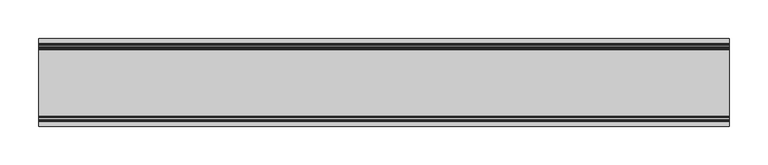
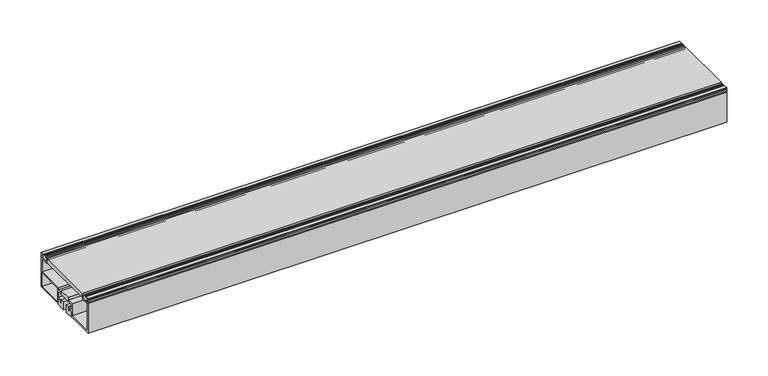
"""IFC4 building model written with IfcOpenShell, lengths in millimetres: proxy geometry, Generic Models 3:Generic Models 1:2:Generic Models 1:2 : Generic Models 3:Generic Models 1:300625:328150:Generic Models 1:2:Generic Models 1:2 : Generic Models 3:Generic Models 1:300625:328150 : Generic Models 3:Generic Models 1:2:Generic Models 1:2 : Generic Models 3:Generic Models 1:300625:328150:4 : Generic Models 3:Generic Models 1:2:Generic Models 1:2 : Generic Models 3:Generic Models 1:300625:328150:Generic Models 1:2:Generic Models 1:2 : Generic Models 3:Generic Models 1:300625:328150 : Generic Models 3:Generic Models 1:2:Generic Models 1:2 : Generic Models 3:Generic Models 1:300625:328150:300962."""

from ifc_helpers import new_model, si_unit, frame, origin, place, context, project, spatial, polyline, outline, extrude, source, transform, mapped, element, save


def generic_models_bcc34015(model_context):
    return source(origin(), model_context, "Body", "SweptSolid", [
        extrude(outline(polyline([(-568050.8100714, 2442.2790126), (-568047.9643932, 2442.2790126), (-568047.9643932, 2445.2228723), (-568043.6663214, 2445.2228723), (-568043.6663214, 2437.3831629), (-568055.5641272, 2435.9222961), (-568055.5641272, 2447.9925532), (-568050.8100714, 2447.9925532), (-568050.8100714, 2442.2790126)])), frame((592836.3867242, 0.0, 0.0), z_axis=(1.0, 0.0, 0.0), x_axis=(0.0, 1.0, 0.0)), (0.0, 0.0, 1.0), 895.35),
        extrude(outline(polyline([(593731.7367242, -568016.9406051), (593731.7367242, -568102.342163), (592836.3867242, -568102.342163), (592836.3867242, -568016.9406051), (593731.7367242, -568016.9406051)])), frame((0.0, 0.0, 2482.8143609), z_axis=(0.0, 0.0, 1.0), x_axis=(1.0, 0.0, 0.0)), (0.0, 0.0, 1.0), 6.35),
        extrude(outline(polyline([(-568002.371855, 2483.7801242), (-568001.9944464, 2482.8143609), (-568007.8625385, 2482.8143609), (-568006.2693218, 2483.6971498), (-568005.2951168, 2484.9385339), (-568005.0923289, 2486.3443102), (-568005.6926824, 2487.6945579), (-568007.0022575, 2488.7780434), (-568007.8625385, 2489.1643609), (-568001.9944464, 2489.1643609), (-568002.371855, 2488.1985977), (-568002.6855411, 2485.9893609), (-568002.371855, 2483.7801242)])), frame((592836.3867242, 0.0, 0.0), z_axis=(1.0, 0.0, 0.0), x_axis=(0.0, 1.0, 0.0)), (0.0, 0.0, 1.0), 895.35),
        extrude(outline(polyline([(-568005.9353019, 2487.3669418), (-568005.4636661, 2485.9893609), (-568005.9353019, 2484.6117801), (-568007.2567959, 2483.507046), (-568009.1664101, 2482.8939648), (-568010.2261661, 2482.8143609), (-568011.285922, 2482.8939648), (-568013.1955363, 2483.507046), (-568014.5170303, 2484.6117801), (-568014.9886661, 2485.9893609), (-568014.5170303, 2487.3669418), (-568013.1955363, 2488.4716759), (-568011.285922, 2489.0847571), (-568010.2261661, 2489.1643609), (-568009.1664101, 2489.0847571), (-568007.2567959, 2488.4716759), (-568005.9353019, 2487.3669418)])), frame((592836.3867242, 0.0, 0.0), z_axis=(1.0, 0.0, 0.0), x_axis=(0.0, 1.0, 0.0)), (0.0, 0.0, 1.0), 895.35),
        extrude(outline(polyline([(-568107.0029708, 2489.0847571), (-568105.0933565, 2488.4716759), (-568103.7718625, 2487.3669418), (-568103.3002267, 2485.9893609), (-568103.7718625, 2484.6117801), (-568105.0933565, 2483.507046), (-568107.0029708, 2482.8939648), (-568108.0627267, 2482.8143609), (-568109.1224826, 2482.8939648), (-568111.0320969, 2483.507046), (-568112.3535909, 2484.6117801), (-568112.8252267, 2485.9893609), (-568112.3535909, 2487.3669418), (-568111.0320969, 2488.4716759), (-568109.1224826, 2489.0847571), (-568108.0627267, 2489.1643609), (-568107.0029708, 2489.0847571)])), frame((592836.3867242, 0.0, 0.0), z_axis=(1.0, 0.0, 0.0), x_axis=(0.0, 1.0, 0.0)), (0.0, 0.0, 1.0), 895.35),
        extrude(outline(polyline([(-568110.4263543, 2489.1643609), (-568111.2866352, 2488.7780434), (-568112.5962104, 2487.6945579), (-568113.1965639, 2486.3443102), (-568112.993776, 2484.9385339), (-568112.019571, 2483.6971498), (-568110.4263543, 2482.8143609), (-568116.2944464, 2482.8143609), (-568115.9170378, 2483.7801242), (-568115.6033517, 2485.9893609), (-568115.9170378, 2488.1985977), (-568116.2944464, 2489.1643609), (-568110.4263543, 2489.1643609)])), frame((592836.3867242, 0.0, 0.0), z_axis=(1.0, 0.0, 0.0), x_axis=(0.0, 1.0, 0.0)), (0.0, 0.0, 1.0), 895.35),
        extrude(outline(polyline([(593731.7367242, -568050.8100714), (593731.7367242, -568067.4788214), (592836.3867242, -568067.4788214), (592836.3867242, -568050.8100714), (593731.7367242, -568050.8100714)])), frame((0.0, 0.0, 2456.2167541), z_axis=(0.0, 0.0, 1.0), x_axis=(1.0, 0.0, 0.0)), (0.0, 0.0, 1.0), 5.5626),
        extrude(outline(polyline([(-568067.4788214, 2442.2790126), (-568067.4788214, 2447.9925532), (-568062.7247655, 2447.9925532), (-568062.7247655, 2435.9222961), (-568074.6225714, 2437.3831629), (-568074.6225714, 2445.2228723), (-568070.3244996, 2445.2228723), (-568070.3244996, 2442.2790126), (-568067.4788214, 2442.2790126)])), frame((592836.3867242, 0.0, 0.0), z_axis=(1.0, 0.0, 0.0), x_axis=(0.0, 1.0, 0.0)), (0.0, 0.0, 1.0), 895.35),
        extrude(outline(polyline([(-568116.2944464, 2482.8162234), (-568103.2073153, 2482.8162234), (-568103.2073153, 2480.9162899), (-568113.7865342, 2480.9162899), (-568113.7865342, 2440.2999335), (-568076.8779936, 2440.2999335), (-568076.8779936, 2458.1166876), (-568043.3108327, 2458.1166876), (-568043.3108327, 2461.7031541), (-568004.5023586, 2461.7031541), (-568004.5023586, 2480.9162899), (-568015.0815775, 2480.9162899), (-568015.0815775, 2482.8162234), (-568001.9944464, 2482.8162234), (-568001.9944464, 2438.4), (-568043.3108327, 2438.4), (-568043.3108327, 2445.6197473), (-568048.4026545, 2445.6197473), (-568048.4026545, 2442.6758876), (-568050.4545827, 2442.6758876), (-568050.4545827, 2447.5956782), (-568043.3108327, 2447.5956782), (-568043.3108327, 2456.2167541), (-568074.9780601, 2456.2167541), (-568074.9780601, 2447.5956782), (-568067.8343101, 2447.5956782), (-568067.8343101, 2442.6758876), (-568069.8862383, 2442.6758876), (-568069.8862383, 2445.6197473), (-568074.9780601, 2445.6197473), (-568074.9780601, 2438.4), (-568116.2944464, 2438.4), (-568116.2944464, 2482.8162234)]), holes=[polyline([(-568041.4108992, 2459.8032206), (-568041.4108992, 2440.2999335), (-568004.5023586, 2440.2999335), (-568004.5023586, 2459.8032206), (-568041.4108992, 2459.8032206)])]), frame((592836.3867242, 0.0, 0.0), z_axis=(1.0, 0.0, 0.0), x_axis=(0.0, 1.0, 0.0)), (0.0, 0.0, 1.0), 895.35),
    ])


if __name__ == "__main__":
    model = new_model("IFC4")
    model_context = context("Model", 3, world=origin())
    ifc_project = project(units=[si_unit("LENGTHUNIT", "METRE", prefix="MILLI")], contexts=[model_context])
    site = spatial("IfcSite", under=ifc_project)
    building = spatial("IfcBuilding", under=site)
    placement = place(None, origin())
    generic_models_shape = generic_models_bcc34015(model_context)
    element("IfcBuildingElementProxy", 1, Name="Generic Models 3:Generic Models 1:2:Generic Models 1:2 : Generic Models 3:Generic Models 1:300625:328150:Generic Models 1:2:Generic Models 1:2 : Generic Models 3:Generic Models 1:300625:328150 : Generic Models 3:Generic Models 1:2:Generic Models 1:2 : Generic Models 3:Generic Models 1:300625:328150:4 : Generic Models 3:Generic Models 1:2:Generic Models 1:2 : Generic Models 3:Generic Models 1:300625:328150:Generic Models 1:2:Generic Models 1:2 : Generic Models 3:Generic Models 1:300625:328150 : Generic Models 3:Generic Models 1:2:Generic Models 1:2 : Generic Models 3:Generic Models 1:300625:328150:300962", ObjectType="Generic Models 3:Generic Models 1:2:Generic Models 1:2 : Generic Models 3:Generic Models 1:300625:328150:Generic Models 1:2:Generic Models 1:2 : Generic Models 3:Generic Models 1:300625:328150 : Generic Models 3:Generic Models 1:2:Generic Models 1:2 : Generic Models 3:Generic Models 1:300625:328150:4 : Generic Models 3:Generic Models 1:2:Generic Models 1:2 : Generic Models 3:Generic Models 1:300625:328150:Generic Models 1:2:Generic Models 1:2 : Generic Models 3:Generic Models 1:300625:328150 : Generic Models 3:Generic Models 1:2:Generic Models 1:2 : Generic Models 3:Generic Models 1:300625:328150:300962", at=placement, inside=building, context=model_context, shape_type="MappedRepresentation", body=[
        mapped(generic_models_shape, transform((0.0, 0.0, 0.0), x_axis=(1.0, 0.0, 0.0), y_axis=(0.0, 1.0, 0.0), z_axis=(0.0, 0.0, 1.0))),
    ])
    save(model, "model.ifc")

# Revit data of these elements
# Type "Generic Models 3:Generic Models 1:2:Generic Models 1:2 : Generic Models 3:Generic Models 1:300625:328150:Generic Models 1:2:Generic Models 1:2 : Generic Models 3:Generic Models 1:300625:328150 : Generic Models 3:Generic Models 1:2:Generic Models 1:2 : Generic Models 3:Generic Models 1:300625:328150:4 : Generic Models 3:Generic Models 1:2:Generic Models 1:2 : Generic Models 3:Generic Models 1:300625:328150:Generic Models 1:2:Generic Models 1:2 : Generic Models 3:Generic Models 1:300625:328150 : Generic Models 3:Generic Models 1:2:Generic Models 1:2 : Generic Models 3:Generic Models 1:300625:328150:300962"
#   NameOverride = "Generic Models 3:Generic Models 1:2:Generic Models 1:2 : Generic Models 3:Generic Models 1:300625:328150:Generic Models 1:2:Generic Models 1:2 : Generic Models 3:Generic Models 1:300625:328150 : Generic Models 3:Generic Models 1:2:Generic Models 1:2 : Generic Models 3:Generic Models 1:300625:328150:300962"
#   ObjectTypeOverride = "Generic Models 1:2:Generic Models 1:2 : Generic Models 3:Generic Models 1:300625:328150 : Generic Models 3:Generic Models 1:2:Generic Models 1:2 : Generic Models 3:Generic Models 1:300625:328150"
#   Reference = "Generic Models 1"
#   Tag = "300962"
# Element 1 (IfcBuildingElementProxy, "Generic Models 3:Generic Models 1:2:Generic Models 1:2 : Generic Models 3:Generic Models 1:300625:328150:Generic Models 1:2:Generic Models 1:2 : Generic Models 3:Generic Models 1:300625:328150 : Generic Models 3:Generic Models 1:2:Generic Models 1:2 : Generic Models 3:Generic Models 1:300625:328150:4 : Generic Models 3:Generic Models 1:2:Generic Models 1:2 : Generic Models 3:Generic Models 1:300625:328150:Generic Models 1:2:Generic Models 1:2 : Generic Models 3:Generic Models 1:300625:328150 : Generic Models 3:Generic Models 1:2:Generic Models 1:2 : Generic Models 3:Generic Models 1:300625:328150:300962")
#   Materials on its faces: "SEALANT & BACKER ROD, IF NECESSARY", "INTERIOR GRADE ALUMINUM STOREFRONT W/ SINGLE GLAZING"
# Materials
#   "SEALANT & BACKER ROD, IF NECESSARY": class "Unassigned", colour RGB 120 120 120, transparency 0, Cost = 0
#   "INTERIOR GRADE ALUMINUM STOREFRONT W/ SINGLE GLAZING": class "Unassigned", colour RGB 244 244 244, transparency 0, Cost = 0
